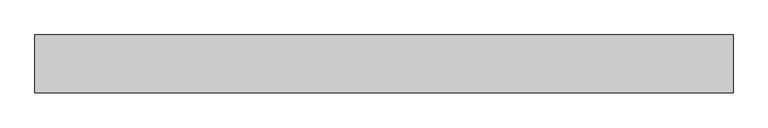
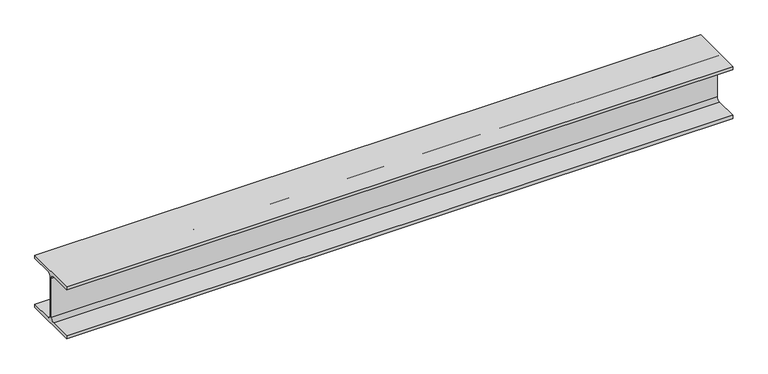
"""IFC4 building model written with IfcOpenShell, lengths in millimetres: beam geometry, 0912_Steel Framing_H-KSD3502 : H_SB_ASB_H-200x200x8x12."""

from ifc_helpers import new_model, si_unit, point, frame, frame_2d, origin, place, context, project, spatial, polyline, circle_curve, trimmed, segment, composite_curve, outline, extrude, source, transform, mapped, element, save


def beam_3646a574(model_context):
    return source(origin(), model_context, "Body", "SweptSolid", [
        extrude(outline(composite_curve([segment(polyline([(100.0, -88.0), (100.0, -100.0), (-100.0, -100.0), (-100.0, -88.0), (-17.0, -88.0)]), True, "CONTINUOUS"), segment(trimmed(circle_curve(frame_2d((-17.0, -75.0)), 13.0), [point((-17.0, -88.0))], [point((-4.0, -75.0))], True, "CARTESIAN"), True, "CONTINUOUS"), segment(polyline([(-4.0, -75.0), (-4.0, 75.0)]), True, "CONTINUOUS"), segment(trimmed(circle_curve(frame_2d((-17.0, 75.0)), 13.0), [point((-4.0, 75.0))], [point((-17.0, 88.0))], True, "CARTESIAN"), True, "CONTINUOUS"), segment(polyline([(-17.0, 88.0), (-100.0, 88.0), (-100.0, 100.0), (100.0, 100.0), (100.0, 88.0), (17.0, 88.0)]), True, "CONTINUOUS"), segment(trimmed(circle_curve(frame_2d((17.0, 75.0)), 13.0), [point((17.0, 88.0))], [point((4.0, 75.0))], True, "CARTESIAN"), True, "CONTINUOUS"), segment(polyline([(4.0, 75.0), (4.0, -75.0)]), True, "CONTINUOUS"), segment(trimmed(circle_curve(frame_2d((17.0, -75.0)), 13.0), [point((4.0, -75.0))], [point((17.0, -88.0))], True, "CARTESIAN"), True, "CONTINUOUS"), segment(polyline([(17.0, -88.0), (100.0, -88.0)]), True, "CONTINUOUS")], self_intersect=False)), frame((-1233.7223186, 0.0, 0.0), z_axis=(1.0, 0.0, 0.0), x_axis=(0.0, 1.0, 0.0)), (0.0, 0.0, 1.0), 2418.936364),
    ])


if __name__ == "__main__":
    model = new_model("IFC4")
    model_context = context("Model", 3, world=origin())
    ifc_project = project(units=[si_unit("LENGTHUNIT", "METRE", prefix="MILLI")], contexts=[model_context])
    site = spatial("IfcSite", under=ifc_project)
    building = spatial("IfcBuilding", under=site)
    placement = place(None, origin())
    beam_shape = beam_3646a574(model_context)
    element("IfcBeam", 1, ObjectType="0912_Steel Framing_H-KSD3502 : H_SB_ASB_H-200x200x8x12", at=placement, inside=building, context=model_context, shape_type="MappedRepresentation", body=[
        mapped(beam_shape, transform((0.0, 0.0, 0.0), x_axis=(1.0, 0.0, 0.0), y_axis=(0.0, 1.0, 0.0), z_axis=(0.0, 0.0, 1.0))),
    ])
    save(model, "model.ifc")

# Revit data of these elements
# Type "0912_Steel Framing_H-KSD3502 : H_SB_ASB_H-200x200x8x12"
#   H_WM Code_1 = "S01AA002-00001 | Main Steel Structure Fabrication Work | Shelter/Building | Medium Steel - Standard (90KG/M>Weight≥30KG/M) | Material: (   )"
#   H_WM Code_2 = "S03AA028-00001 | Main Steel Structure Erection Work | Shelter/Building | Medium Steel (90KG/M>Weight≥30KG/M) | Material: (   )"
#   H_WM Code_3 = "S01AA010-00001 | Main Steel Structure Fabrication Work | Shelter/Building | Steel Painting/Coating | for Non-Fireproofed Steel Surface, Surface Preparation, Primer, Second & Final Coat | Material: (   )"
#   H_Q'ty Cal Type Tag = "SB-Q2"
#   Width = 20.0 cm
#   Web Thickness = 0.8 cm
#   Web Fillet = 1.3 cm
#   Warping Constant = 141000.0 cm⁶
#   W = 0
#   Torsional Moment of Inertia = 26.2485 cm⁴
#   Section Area = 63.53 cm²
#   Plastic Modulus weak axis = 244.0 cm³
#   Plastic Modulus strong axis = 525.0 cm³
#   Perimeter = 1.16 m²/m
#   Nominal Weight = 49.90 kgf/m
#   Moment of Inertia weak axis = 1600.00 cm⁴
#   Moment of Inertia strong axis = 4720.00 cm⁴
#   Height = 20.0 cm
#   Flange Thickness = 1.2 cm
#   Elastic Modulus weak axis = 160.0 cm³
#   Elastic Modulus strong axis = 472.0 cm³
#   Centroid Vertical = 10.0 cm
#   Centroid Horizontal = 10.0 cm
#   Ix = 47200000
#   Length [instance default] = 1.5240 m
#   Zx = 525000
#   b = 0.2000 m
#   h = 0.2000 m
#   r = 0.0130 m
#   s = 0.0080 m
#   t = 0.0120 m
#   A = 0.006353 m²
#   Structural Material [instance default] = Steel, 45-345
#   Assembly Code = ""
# Element 1 (IfcBeam, "0912_Steel Framing_H-KSD3502 : H_SB_ASB_H-200x200x8x12")
#   Structural Material = none
# Materials
#   "Steel, 45-345": class "Metal", colour RGB 189 187 185, transparency 0, Description = "Steel 345 MPa", Cost = 0
